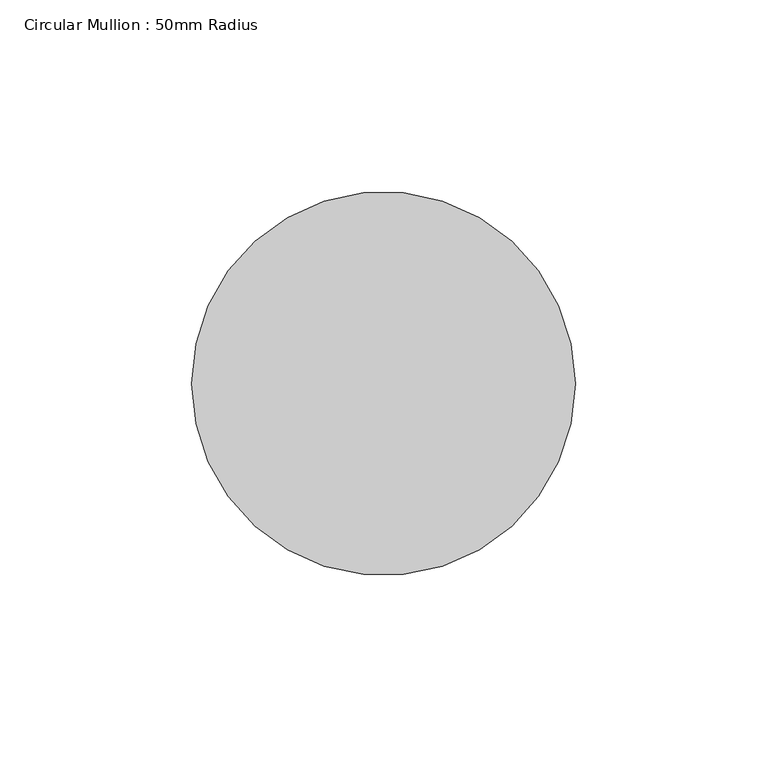
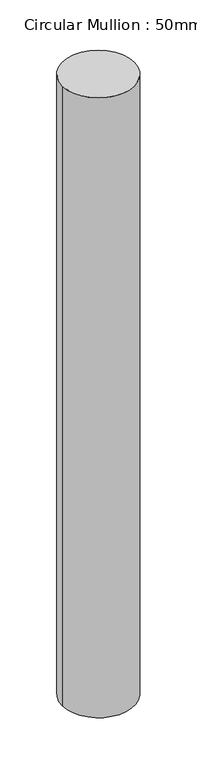
"""IFC4 building model written with IfcOpenShell, lengths in millimetres: member geometry, Circular Mullion : 50mm Radius."""

from ifc_helpers import new_model, si_unit, point, frame, origin, origin_2d, place, context, project, spatial, circle_curve, trimmed, segment, composite_curve, outline, extrude, source, transform, mapped, element, save


def circular_mullion_50mm_radius_20605bbf(model_context):
    return source(origin(), model_context, "Body", "SweptSolid", [
        extrude(outline(composite_curve([segment(trimmed(circle_curve(origin_2d(), 50.0), [point((50.0, 0.0))], [point((-50.0, 0.0))], False, "CARTESIAN"), True, "CONTINUOUS"), segment(trimmed(circle_curve(origin_2d(), 50.0), [point((-50.0, 0.0))], [point((50.0, 0.0))], False, "CARTESIAN"), True, "CONTINUOUS")], self_intersect=False)), frame((0.0, 0.0, -910.3224864), z_axis=(0.0, 0.0, 1.0), x_axis=(1.0, 0.0, 0.0)), (0.0, 0.0, 1.0), 910.3224864),
    ])


if __name__ == "__main__":
    model = new_model("IFC4")
    model_context = context("Model", 3, world=origin())
    ifc_project = project(units=[si_unit("LENGTHUNIT", "METRE", prefix="MILLI")], contexts=[model_context])
    site = spatial("IfcSite", under=ifc_project)
    building = spatial("IfcBuilding", under=site)
    placement = place(None, origin())
    circular_mullion_50mm_radius_shape = circular_mullion_50mm_radius_20605bbf(model_context)
    element("IfcMember", 1, ObjectType="Circular Mullion : 50mm Radius", at=placement, inside=building, context=model_context, shape_type="MappedRepresentation", body=[
        mapped(circular_mullion_50mm_radius_shape, transform((0.0, 0.0, 0.0), x_axis=(1.0, 0.0, 0.0), y_axis=(0.0, 1.0, 0.0), z_axis=(0.0, 0.0, 1.0))),
    ])
    save(model, "model.ifc")

# Revit data of these elements
# Type "Circular Mullion : 50mm Radius"
#   built-in parameter 1007350 = 0.164042 (stored number, unit not read)
# Element 1 (IfcMember, "Circular Mullion : 50mm Radius")
#   Materials on its faces: "Aluminium"
# Materials
#   "Aluminium": class "Metal", colour RGB 247 247 247, transparency 0, Description = "Aluminium 6061", Cost = 0
